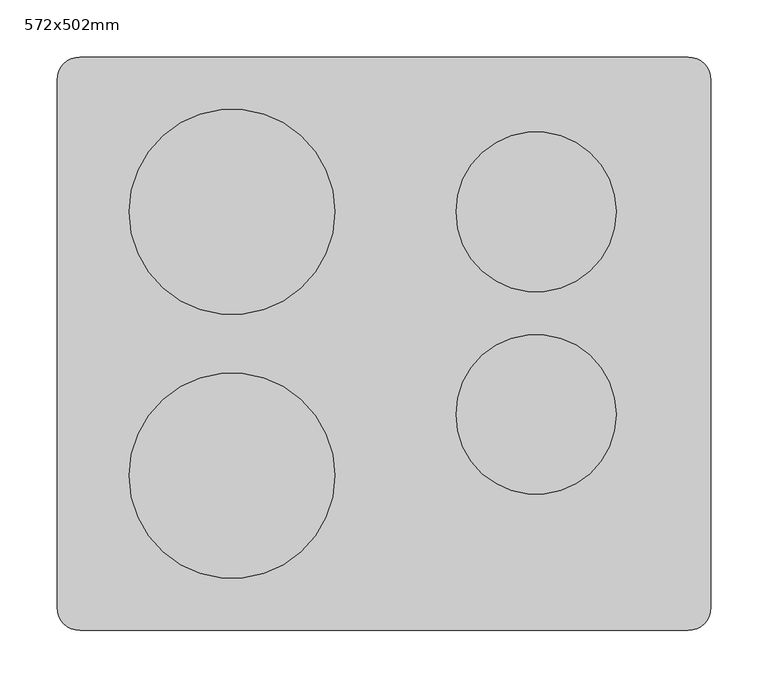
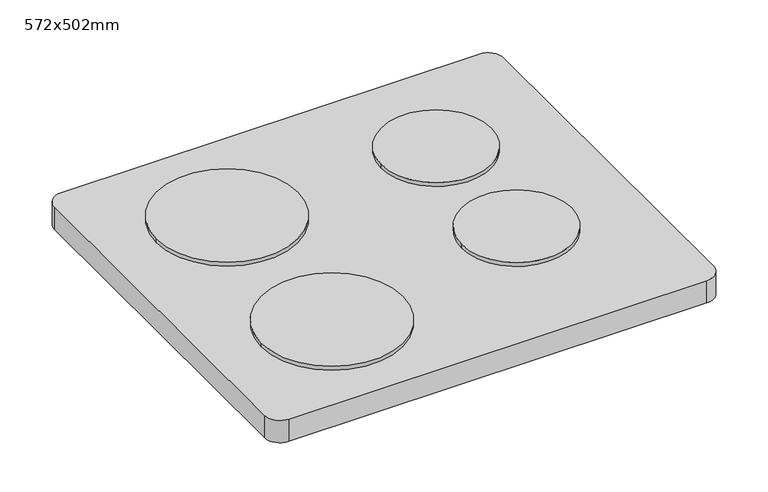
"""IFC4 building model written with IfcOpenShell, lengths in millimetres: proxy geometry, Specialty_Equipment_Electric_Hob : 572x502mm."""

import ifcopenshell
import ifcopenshell.guid

model = None  # the IFC model being written
_history = None  # IfcOwnerHistory: only IFC2X3 demands one
_inside = {}  # id of a spatial element -> (the spatial element, [elements in it])
_under = {}  # id of a project, library or spatial element -> (it, [spatial elements below it])
_declared = {}  # id of a project -> (the project, [libraries it declares])
_typed = {}  # id of a type object -> (the type object, [elements of that type])
_made_of = {}  # id of a material, layer set ... -> (it, [elements and type objects made of it])


def new_model(schema):
    """Start an empty IFC model of exactly this schema.

    Asked for "IFC4X3", IfcOpenShell would pick the latest addendum, in which some entities
    have other attributes; the version numbers below select the first issue.
    IFC2X3 requires an IfcOwnerHistory on every rooted entity: one is made here for all.
    """
    global model, _history
    if schema == "IFC4X3":
        model = ifcopenshell.file(schema_version=(4, 3, 0, 0))
    else:
        model = ifcopenshell.file(schema=schema)
    _inside.clear()
    _under.clear()
    _declared.clear()
    _typed.clear()
    _made_of.clear()
    _history = None
    if model.schema == "IFC2X3":
        org = make("IfcOrganization", Name="unknown")
        user = make(
            "IfcPersonAndOrganization",
            ThePerson=make("IfcPerson", FamilyName="unknown"),
            TheOrganization=org,
        )
        app = make(
            "IfcApplication",
            ApplicationDeveloper=org,
            Version="unknown",
            ApplicationFullName="unknown",
            ApplicationIdentifier="unknown",
        )
        _history = make(
            "IfcOwnerHistory",
            OwningUser=user,
            OwningApplication=app,
            ChangeAction="ADDED",
            CreationDate=0,
        )
    return model


def make(cls, **values):
    """One entity of the class cls with the attributes given. An attribute that is None is left unset."""
    return model.create_entity(
        cls, **{name: value for name, value in values.items() if value is not None}
    )


def rooted(cls, **values):
    """An entity with a GlobalId (a new one), such as an element, a storey or a relation."""
    return make(cls, GlobalId=ifcopenshell.guid.new(), OwnerHistory=_history, **values)


def si_unit(unit_type, name, prefix=None):
    """IfcSIUnit, for example si_unit("LENGTHUNIT", "METRE", prefix="MILLI")."""
    return make("IfcSIUnit", UnitType=unit_type, Prefix=prefix, Name=name)


def assignment(units):
    """IfcUnitAssignment: the units of a project."""
    return None if units is None else make("IfcUnitAssignment", Units=units)


def point(xyz):
    """IfcCartesianPoint."""
    return None if xyz is None else make("IfcCartesianPoint", Coordinates=xyz)


def direction(xyz):
    """IfcDirection."""
    return None if xyz is None else make("IfcDirection", DirectionRatios=xyz)


def frame(location, z_axis=None, x_axis=None):
    """IfcAxis2Placement3D, a coordinate frame: its origin and axes. An axis left out is left unset."""
    return make(
        "IfcAxis2Placement3D",
        Location=point(location),
        Axis=direction(z_axis),
        RefDirection=direction(x_axis),
    )


def frame_2d(location, x_axis=None):
    """IfcAxis2Placement2D, a coordinate frame in the plane: its origin and x axis."""
    return make(
        "IfcAxis2Placement2D", Location=point(location), RefDirection=direction(x_axis)
    )


def origin():
    """The frame at (0, 0, 0) with its axes left unset."""
    return frame((0.0, 0.0, 0.0))


def origin_with_axes():
    """The frame at (0, 0, 0) with the z axis (0, 0, 1) and the x axis (1, 0, 0) written out."""
    return frame((0.0, 0.0, 0.0), z_axis=(0.0, 0.0, 1.0), x_axis=(1.0, 0.0, 0.0))


def place(relative_to, where):
    """IfcLocalPlacement: puts the frame where relative to a parent placement (None: the world)."""
    return make(
        "IfcLocalPlacement", PlacementRelTo=relative_to, RelativePlacement=where
    )


def context(
    kind, dimensions, precision=None, world=None, true_north=None, identifier=None
):
    """IfcGeometricRepresentationContext, for example the 3D "Model" context."""
    return make(
        "IfcGeometricRepresentationContext",
        ContextIdentifier=identifier,
        ContextType=kind,
        CoordinateSpaceDimension=dimensions,
        Precision=precision,
        WorldCoordinateSystem=world,
        TrueNorth=true_north,
    )


def project(units=None, contexts=None):
    """IfcProject with its units and contexts."""
    return rooted(
        "IfcProject",
        Name="project",
        RepresentationContexts=contexts,
        UnitsInContext=assignment(units),
    )


def spatial(cls, under=None, at=None, **own):
    """A site, building, storey or space (cls), placed at a placement, below another one or the project."""
    s = rooted(cls, ObjectPlacement=at, **own)
    if under is not None:
        _under.setdefault(under.id(), (under, []))[1].append(s)
    return s


def polyline(points):
    """IfcPolyline through the points."""
    return make("IfcPolyline", Points=[point(p) for p in points])


def circle_curve(where, radius):
    """IfcCircle in the frame where."""
    return make("IfcCircle", Position=where, Radius=radius)


def trimmed(basis, trim1, trim2, sense, master):
    """IfcTrimmedCurve: the piece of a basis curve between two trims."""
    return make(
        "IfcTrimmedCurve",
        BasisCurve=basis,
        Trim1=trim1,
        Trim2=trim2,
        SenseAgreement=sense,
        MasterRepresentation=master,
    )


def segment(curve, same_sense, transition):
    """IfcCompositeCurveSegment."""
    return make(
        "IfcCompositeCurveSegment",
        Transition=transition,
        SameSense=same_sense,
        ParentCurve=curve,
    )


def composite_curve(segments, self_intersect=None):
    """IfcCompositeCurve: segments joined end to end."""
    return make("IfcCompositeCurve", Segments=segments, SelfIntersect=self_intersect)


def outline(outer, holes=None, kind="AREA"):
    """IfcArbitraryClosedProfileDef: a profile drawn as a closed curve; with holes, ...WithVoids."""
    if holes is None:
        return make("IfcArbitraryClosedProfileDef", ProfileType=kind, OuterCurve=outer)
    return make(
        "IfcArbitraryProfileDefWithVoids",
        ProfileType=kind,
        OuterCurve=outer,
        InnerCurves=holes,
    )


def extrude(swept, where, along, depth):
    """IfcExtrudedAreaSolid: the profile swept, set in the frame where, extruded along a direction by depth."""
    return make(
        "IfcExtrudedAreaSolid",
        SweptArea=swept,
        Position=where,
        ExtrudedDirection=direction(along),
        Depth=depth,
    )


def shape(context_of_items, identifier, shape_type, items):
    """IfcShapeRepresentation: the items that make up one representation, for example the "Body"."""
    return make(
        "IfcShapeRepresentation",
        ContextOfItems=context_of_items,
        RepresentationIdentifier=identifier,
        RepresentationType=shape_type,
        Items=items,
    )


def source(mapping_origin, context_of_items, identifier, shape_type, items):
    """IfcRepresentationMap: a shape defined once, which mapped items show again and again."""
    return make(
        "IfcRepresentationMap",
        MappingOrigin=mapping_origin,
        MappedRepresentation=shape(context_of_items, identifier, shape_type, items),
    )


def transform(
    local_origin,
    x_axis=None,
    y_axis=None,
    z_axis=None,
    scale=None,
    scale2=None,
    scale3=None,
    uniform=True,
):
    """IfcCartesianTransformationOperator3D, or its non-uniform kind. x_axis, y_axis, z_axis: its Axis1, 2, 3."""
    if uniform:
        return make(
            "IfcCartesianTransformationOperator3D",
            Axis1=direction(x_axis),
            Axis2=direction(y_axis),
            LocalOrigin=point(local_origin),
            Scale=scale,
            Axis3=direction(z_axis),
        )
    return make(
        "IfcCartesianTransformationOperator3DnonUniform",
        Axis1=direction(x_axis),
        Axis2=direction(y_axis),
        LocalOrigin=point(local_origin),
        Scale=scale,
        Axis3=direction(z_axis),
        Scale2=scale2,
        Scale3=scale3,
    )


def mapped(mapping_source, mapping_target):
    """IfcMappedItem: shows the shape of a source again, moved by a transform."""
    return make(
        "IfcMappedItem", MappingSource=mapping_source, MappingTarget=mapping_target
    )


def made_of(thing, what):
    """Note that an element or type object is made of a material, layer set ...; save() writes the relation."""
    if what is not None:
        _made_of.setdefault(what.id(), (what, []))[1].append(thing)
    return thing


def element(
    cls,
    number,
    at=None,
    inside=None,
    cuts=None,
    type_object=None,
    material=None,
    context=None,
    identifier="Body",
    shape_type=None,
    held_by="IfcProductDefinitionShape",
    body=None,
    shapes=None,
    **own,
):
    """One element of the class cls, such as IfcWall. Its Tag is "e" and its number.

    at: its placement. inside: the storey or other place that contains it. cuts: it is an
    opening in that element (IfcRelVoidsElement). A single representation is given by context,
    identifier, shape_type and body (its items); several are given by shapes. held_by: the class
    of the entity that holds the representations. save() writes the other relations.
    """
    e = rooted(cls, Tag="e%d" % number, ObjectPlacement=at, **own)
    if body is not None:
        shapes = [shape(context, identifier, shape_type, body)]
    if shapes is not None:
        e.Representation = make(held_by, Representations=shapes)
    if inside is not None:
        _inside.setdefault(inside.id(), (inside, []))[1].append(e)
    if cuts is not None:
        rooted(
            "IfcRelVoidsElement", RelatingBuildingElement=cuts, RelatedOpeningElement=e
        )
    if type_object is not None:
        _typed.setdefault(type_object.id(), (type_object, []))[1].append(e)
    return made_of(e, material)


def aggregate(whole, parts):
    """IfcRelAggregates: a whole, such as a stair, and the parts it consists of."""
    return rooted("IfcRelAggregates", RelatingObject=whole, RelatedObjects=parts)


def save(model, path):
    """Write the relations noted so far, then the file.

    IfcRelAggregates (storeys below a building ...), IfcRelContainedInSpatialStructure (elements
    in a storey), IfcRelDefinesByType, IfcRelAssociatesMaterial and IfcRelDeclares: one each for
    every whole, place, type object, material and project.
    """
    for whole, parts in _under.values():
        aggregate(whole, parts)
    for where, things in _inside.values():
        rooted(
            "IfcRelContainedInSpatialStructure",
            RelatedElements=things,
            RelatingStructure=where,
        )
    for kind, things in _typed.values():
        rooted("IfcRelDefinesByType", RelatedObjects=things, RelatingType=kind)
    for what, things in _made_of.values():
        rooted("IfcRelAssociatesMaterial", RelatedObjects=things, RelatingMaterial=what)
    for by, libraries in _declared.values():
        rooted("IfcRelDeclares", RelatingContext=by, RelatedDefinitions=libraries)
    model.write(path)


def proxy_572x502mm_ba399a0f(model_context):
    return source(origin(), model_context, "Body", "SweptSolid", [
        extrude(outline(composite_curve([segment(trimmed(circle_curve(frame_2d((-112.0, 115.5)), 90.0), [point((-202.0, 115.5))], [point((-22.0, 115.5))], False, "CARTESIAN"), True, "CONTINUOUS"), segment(trimmed(circle_curve(frame_2d((-112.0, 115.5)), 90.0), [point((-22.0, 115.5))], [point((-202.0, 115.5))], False, "CARTESIAN"), True, "CONTINUOUS")], self_intersect=False)), frame((0.0, 0.0, 30.0), z_axis=(0.0, 0.0, 1.0), x_axis=(1.0, 0.0, 0.0)), (0.0, 0.0, 1.0), 5.0),
        extrude(outline(composite_curve([segment(trimmed(circle_curve(frame_2d((-112.0, -115.5)), 90.0), [point((-202.0, -115.5))], [point((-22.0, -115.5))], False, "CARTESIAN"), True, "CONTINUOUS"), segment(trimmed(circle_curve(frame_2d((-112.0, -115.5)), 90.0), [point((-22.0, -115.5))], [point((-202.0, -115.5))], False, "CARTESIAN"), True, "CONTINUOUS")], self_intersect=False)), frame((0.0, 0.0, 30.0), z_axis=(0.0, 0.0, 1.0), x_axis=(1.0, 0.0, 0.0)), (0.0, 0.0, 1.0), 5.0),
        extrude(outline(composite_curve([segment(trimmed(circle_curve(frame_2d((154.0, 115.5)), 70.0), [point((84.0, 115.5))], [point((224.0, 115.5))], False, "CARTESIAN"), True, "CONTINUOUS"), segment(trimmed(circle_curve(frame_2d((154.0, 115.5)), 70.0), [point((224.0, 115.5))], [point((84.0, 115.5))], False, "CARTESIAN"), True, "CONTINUOUS")], self_intersect=False)), frame((0.0, 0.0, 30.0), z_axis=(0.0, 0.0, 1.0), x_axis=(1.0, 0.0, 0.0)), (0.0, 0.0, 1.0), 5.0),
        extrude(outline(composite_curve([segment(trimmed(circle_curve(frame_2d((154.0, -61.8682566)), 70.0), [point((84.0, -61.8682566))], [point((224.0, -61.8682566))], False, "CARTESIAN"), True, "CONTINUOUS"), segment(trimmed(circle_curve(frame_2d((154.0, -61.8682566)), 70.0), [point((224.0, -61.8682566))], [point((84.0, -61.8682566))], False, "CARTESIAN"), True, "CONTINUOUS")], self_intersect=False)), frame((0.0, 0.0, 30.0), z_axis=(0.0, 0.0, 1.0), x_axis=(1.0, 0.0, 0.0)), (0.0, 0.0, 1.0), 5.0),
        extrude(outline(composite_curve([segment(polyline([(287.0, -251.0), (-245.0, -251.0)]), True, "CONTINUOUS"), segment(trimmed(circle_curve(frame_2d((-245.0, -231.0)), 20.0), [point((-245.0, -251.0))], [point((-265.0, -231.0))], False, "CARTESIAN"), True, "CONTINUOUS"), segment(polyline([(-265.0, -231.0), (-265.0, 231.0)]), True, "CONTINUOUS"), segment(trimmed(circle_curve(frame_2d((-245.0, 231.0)), 20.0), [point((-265.0, 231.0))], [point((-245.0, 251.0))], False, "CARTESIAN"), True, "CONTINUOUS"), segment(polyline([(-245.0, 251.0), (287.0, 251.0)]), True, "CONTINUOUS"), segment(trimmed(circle_curve(frame_2d((287.0, 231.0)), 20.0), [point((287.0, 251.0))], [point((307.0, 231.0))], False, "CARTESIAN"), True, "CONTINUOUS"), segment(polyline([(307.0, 231.0), (307.0, -231.0)]), True, "CONTINUOUS"), segment(trimmed(circle_curve(frame_2d((287.0, -231.0)), 20.0), [point((307.0, -231.0))], [point((287.0, -251.0))], False, "CARTESIAN"), True, "CONTINUOUS")], self_intersect=False)), origin_with_axes(), (0.0, 0.0, 1.0), 30.0),
    ])


if __name__ == "__main__":
    model = new_model("IFC4")
    model_context = context("Model", 3, world=origin())
    ifc_project = project(units=[si_unit("LENGTHUNIT", "METRE", prefix="MILLI")], contexts=[model_context])
    site = spatial("IfcSite", under=ifc_project)
    building = spatial("IfcBuilding", under=site)
    placement = place(None, origin())
    proxy_572x502mm_shape = proxy_572x502mm_ba399a0f(model_context)
    element("IfcBuildingElementProxy", 1, Name="Specialty_Equipment_Electric_Hob : 572x502mm", ObjectType="Specialty_Equipment_Electric_Hob : 572x502mm", at=placement, inside=building, context=model_context, shape_type="MappedRepresentation", body=[
        mapped(proxy_572x502mm_shape, transform((0.0, 0.0, 0.0), x_axis=(1.0, 0.0, 0.0), y_axis=(0.0, 1.0, 0.0), z_axis=(0.0, 0.0, 1.0))),
    ])
    save(model, "model.ifc")

# Revit data of these elements
# Type "Specialty_Equipment_Electric_Hob : 572x502mm"
#   Keynote = "N"
#   Depth = 502 mm
#   Width = 572 mm
#   Material Hob = Metal - Stainless Steel
#   Default Elevation = 0
# Element 1 (IfcBuildingElementProxy, "Specialty_Equipment_Electric_Hob : 572x502mm")
#   Materials on its faces: "Metal - Paint Finish - Dark Gray, Matte", "Metal - Stainless Steel"
# Materials
#   "Metal - Stainless Steel": class "Metal", colour RGB 173 173 173, transparency 0
#   "Metal - Paint Finish - Dark Gray, Matte": class "Paint", colour RGB 98 98 98, transparency 0
